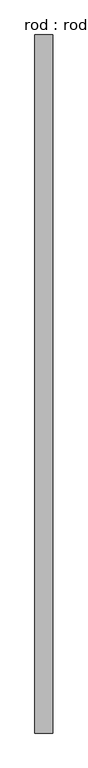
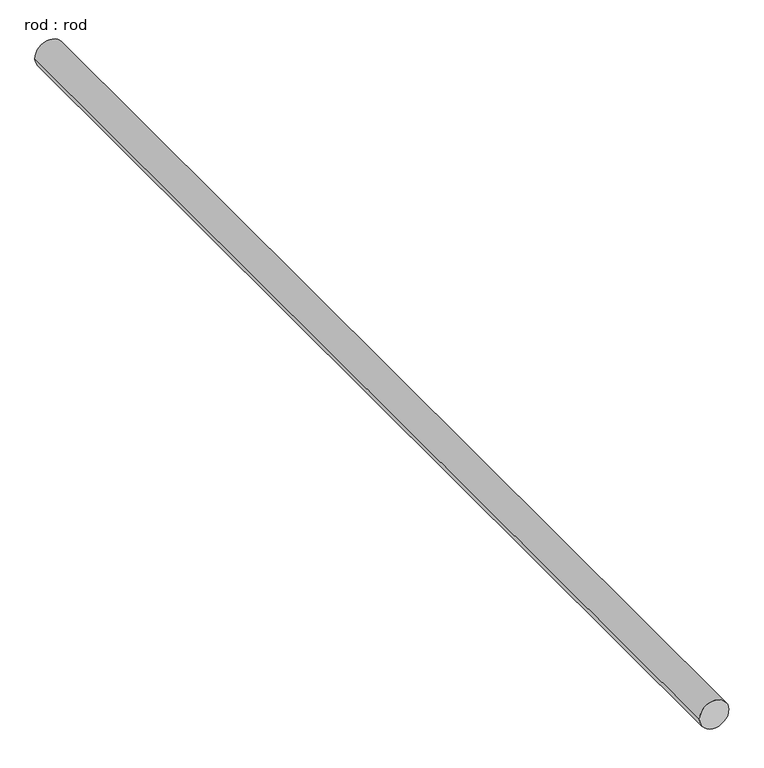
"""IFC4 building model written with IfcOpenShell, lengths in millimetres: proxy geometry, rod : rod."""

from ifc_helpers import new_model, si_unit, point, frame, frame_2d, origin, place, context, project, spatial, circle_curve, trimmed, segment, composite_curve, outline, extrude, source, transform, mapped, element, save


def rod_rod_6f444b85(model_context):
    return source(origin(), model_context, "Body", "SweptSolid", [
        extrude(outline(composite_curve([segment(trimmed(circle_curve(frame_2d((0.0108462, 0.0)), 200.0), [point((0.0108462, 200.0))], [point((0.0108462, -200.0))], False, "CARTESIAN"), True, "CONTINUOUS"), segment(trimmed(circle_curve(frame_2d((0.0108462, 0.0)), 200.0), [point((0.0108462, -200.0))], [point((0.0108462, 200.0))], False, "CARTESIAN"), True, "CONTINUOUS")], self_intersect=False)), frame((0.0, -3750.8042019, 0.0), z_axis=(0.0, 1.0, 0.0), x_axis=(0.0, 0.0, 1.0)), (0.0, 0.0, 1.0), 15687.0656345),
    ])


if __name__ == "__main__":
    model = new_model("IFC4")
    model_context = context("Model", 3, world=origin())
    ifc_project = project(units=[si_unit("LENGTHUNIT", "METRE", prefix="MILLI")], contexts=[model_context])
    site = spatial("IfcSite", under=ifc_project)
    building = spatial("IfcBuilding", under=site)
    placement = place(None, origin())
    rod_rod_shape = rod_rod_6f444b85(model_context)
    element("IfcBuildingElementProxy", 1, Name="rod : rod", ObjectType="rod : rod", at=placement, inside=building, context=model_context, shape_type="MappedRepresentation", body=[
        mapped(rod_rod_shape, transform((0.0, 0.0, 0.0), x_axis=(1.0, 0.0, 0.0), y_axis=(0.0, 1.0, 0.0), z_axis=(0.0, 0.0, 1.0))),
    ])
    save(model, "model.ifc")

# Revit data of these elements
# Type "rod : rod"
#   Default Elevation = 0
